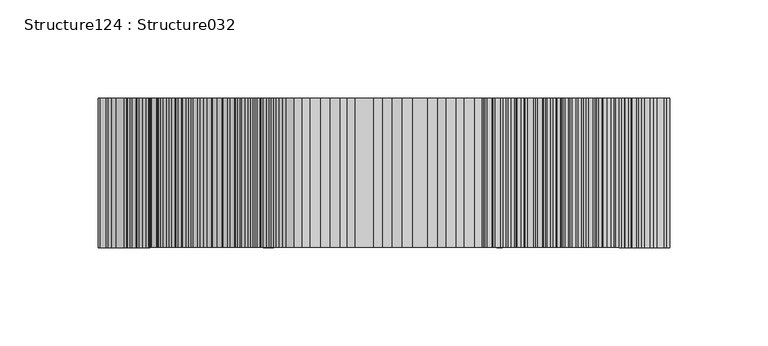
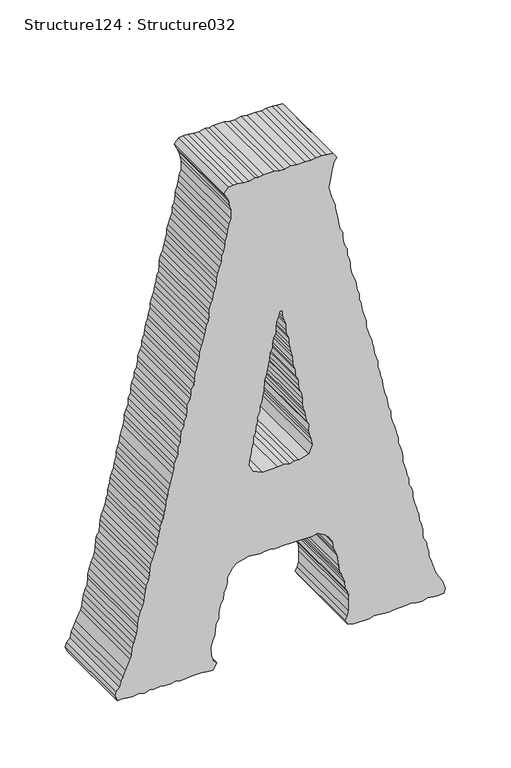
"""IFC4 building model written with IfcOpenShell, lengths in millimetres: proxy geometry, Structure124 : Structure032."""

from ifc_helpers import new_model, si_unit, frame, origin, place, context, project, spatial, polyline, outline, extrude, source, transform, mapped, element, save


def structure124_structure032_16c82b9b(model_context):
    return source(origin(), model_context, "Body", "SweptSolid", [
        extrude(outline(polyline([(3818.8310229, -39965.9490603), (3814.7296538, -39965.9490603), (3811.2043377, -39967.1091894), (3805.9476534, -39969.4487027), (3801.8462843, -39969.4487027), (3795.960595, -39970.0279649), (3791.8865042, -39972.3899428), (3787.7867397, -39972.3899428), (3783.0868532, -39974.7310607), (3777.8285642, -39975.3327874), (3773.11905, -39975.3327874), (3769.6274306, -39977.6498363), (3763.759392, -39977.6498363), (3759.6596275, -39979.4100874), (3755.559863, -39981.1719432), (3750.8583719, -39981.1719432), (3746.1745313, -39982.3529321), (3737.400554, -39984.669981), (3732.1149867, -39985.8509699), (3727.4311462, -39987.0319588), (3723.3313817, -39988.2129477), (3718.6571688, -39988.2129477), (3713.3555556, -39989.9748034), (3709.2718371, -39990.5540657), (3704.5879966, -39992.2918523), (3701.0723082, -39993.4728412), (3695.786741, -39994.0521035), (3690.512406, -39995.8139592), (3685.8285655, -39995.8139592), (3682.8857208, -39996.9949481), (3677.6274319, -39998.175937), (3672.9435914, -39999.9137237), (3668.8261762, -40001.6739748), (3664.1423357, -40002.253237), (3660.0682449, -40002.8549637), (3654.1841602, -40003.4358305), (3650.1004418, -40005.7978084), (3645.9830266, -40006.3770706), (3641.2991861, -40006.9338683), (3636.0408972, -40007.535595), (3631.915459, -40008.7165839), (3627.8397636, -40010.4768351), (3622.555801, -40012.2386908), (3617.2718384, -40013.3972153), (3613.772196, -40013.3972153), (3607.8961343, -40013.9989419), (3604.3964919, -40015.7367286), (3600.2967274, -40016.9177175), (3595.5872132, -40018.0778466), (3589.7544759, -40018.6795733), (3586.2115092, -40019.8605622), (3577.4535778, -40023.9378622), (3572.1423369, -40026.3014446), (3568.6426945, -40028.0616957), (3563.366755, -40029.1977557), (3560.441561, -40032.1389958), (3556.3417965, -40033.3215893), (3551.6675836, -40031.5597335), (3551.6675836, -40026.8807068), (3551.0658569, -40022.1776111), (3550.4833855, -40018.0778466), (3551.6675836, -40012.817953), (3550.4833855, -40007.535595), (3551.6675836, -40002.8549637), (3551.0658569, -39999.3344615), (3551.6675836, -39993.4728412), (3551.0658569, -39989.9748034), (3551.0658569, -39984.0907187), (3551.6675836, -39979.9893497), (3551.0658569, -39975.9120496), (3551.0658569, -39971.2089539), (3551.6675836, -39966.5299271), (3551.6675836, -39957.1462001), (3551.0658569, -39952.4671733), (3550.4833855, -39947.1848153), (3556.3417965, -39943.6851729), (3559.2669905, -39946.6055531), (3565.1254015, -39948.3658043), (3572.7440636, -39948.9450665), (3578.6104977, -39947.1848153), (3582.7102621, -39945.4470287), (3587.3860796, -39944.845302), (3592.0955938, -39944.2660398), (3596.7698067, -39941.9024573), (3601.4536473, -39941.9024573), (3604.9709403, -39941.3231951), (3610.2292293, -39940.1422062), (3613.772196, -39937.8251573), (3619.6145609, -39937.2458951), (3622.555801, -39935.4615749), (3627.8397636, -39934.3030505), (3633.0980525, -39934.3030505), (3639.5405396, -39929.6240237), (3643.0578326, -39926.1019169), (3644.8245022, -39919.0593077), (3645.9830266, -39915.5612699), (3645.4262289, -39909.6771853), (3644.8245022, -39905.5982806), (3645.4262289, -39900.9192539), (3645.9830266, -39896.2161581), (3644.8245022, -39892.1163937), (3645.4262289, -39886.8340357), (3645.4262289, -39874.531533), (3644.8245022, -39868.6699128), (3644.8245022, -39859.2877903), (3645.9830266, -39854.6087636), (3642.4833842, -39848.1678811), (3638.9580681, -39844.066512), (3633.0980525, -39841.1477365), (3627.2396415, -39839.9667475), (3622.555801, -39838.2048918), (3619.6145609, -39837.0239029), (3609.0723094, -39835.8653785), (3604.3964919, -39834.6843895), (3600.2967274, -39833.5258651), (3596.1953583, -39831.7640094), (3592.0955938, -39830.5830205), (3586.2115092, -39830.0037582), (3582.7102621, -39828.2435071), (3578.6104977, -39827.0625182), (3573.9266571, -39827.0625182), (3563.9412034, -39827.0625182), (3559.2669905, -39828.2435071), (3555.7416744, -39830.0037582), (3551.6675836, -39827.6642449), (3550.4833855, -39822.3818869), (3550.4833855, -39808.9208598), (3551.6675836, -39804.7986308), (3551.0658569, -39799.5387373), (3550.4833855, -39794.858106), (3550.4833855, -39790.735877), (3551.0658569, -39784.8967213), (3551.0658569, -39780.7969568), (3551.6675836, -39776.093861), (3551.6675836, -39771.9924919), (3550.4833855, -39767.3134652), (3550.4833855, -39762.0311072), (3551.6675836, -39757.3504759), (3551.0658569, -39752.0697225), (3550.4833855, -39748.5700801), (3551.0658569, -39742.7084599), (3555.1848766, -39741.5274709), (3560.441561, -39743.2893267), (3563.366755, -39744.4478511), (3568.6426945, -39747.9683534), (3572.1423369, -39749.7286045), (3576.2693797, -39751.5129247), (3586.2115092, -39754.4092358), (3590.3289243, -39756.169487), (3594.4286888, -39756.169487), (3599.1125293, -39757.3504759), (3604.3964919, -39758.5330694), (3608.4705827, -39760.8501183), (3612.5976255, -39761.451845), (3617.2718384, -39761.451845), (3622.555801, -39762.6328339), (3627.2396415, -39764.393085), (3632.5155811, -39764.9723472), (3636.0408972, -39766.1549407), (3640.114988, -39767.3134652), (3645.4262289, -39769.0737163), (3650.6845178, -39770.2322408), (3655.3587307, -39770.2322408), (3659.4584952, -39771.4132297), (3663.5598643, -39773.7768121), (3668.8261762, -39773.7768121), (3673.5276674, -39775.5145988), (3677.0449605, -39776.093861), (3682.8857208, -39777.8541121), (3686.4030139, -39779.035101), (3691.0868544, -39779.035101), (3695.2122926, -39779.6143633), (3699.8881101, -39780.7969568), (3705.7545441, -39783.1140057), (3710.4560353, -39783.1140057), (3714.5301261, -39784.2949946), (3718.0554422, -39785.4759835), (3723.3313817, -39786.6569724), (3727.4311462, -39788.4188281), (3732.7167134, -39789.5773526), (3737.9750024, -39789.5773526), (3740.9162424, -39791.3376037), (3745.6000829, -39792.4961281), (3751.4424479, -39793.0978548), (3756.1423345, -39794.858106), (3759.6596275, -39796.0406995), (3764.3611187, -39796.6199617), (3769.0176809, -39797.1767595), (3774.3032481, -39798.9370106), (3777.8285642, -39799.5387373), (3783.0868532, -39801.2989884), (3788.3611881, -39801.2989884), (3791.8865042, -39802.4799773), (3797.1463977, -39804.2193686), (3801.8462843, -39804.7986308), (3806.5317294, -39805.9796197), (3810.0474179, -39806.5588819), (3815.3313805, -39808.9208598), (3820.015221, -39810.0809888), (3824.1149855, -39811.2619777), (3829.374879, -39811.2619777), (3837.6000817, -39814.1807533), (3842.8583706, -39815.3617422), (3846.9757858, -39815.9410044), (3851.6612309, -39817.7028602), (3856.9179152, -39817.7028602), (3861.0192843, -39819.4406468), (3866.3032469, -39820.0423735), (3869.8189354, -39820.6216357), (3873.9203044, -39822.3818869), (3878.5784713, -39824.142138), (3883.8881076, -39825.3247315), (3888.5623205, -39825.3247315), (3892.6636896, -39826.5057204), (3897.3475301, -39828.2435071), (3902.6314927, -39828.2435071), (3906.1487857, -39830.5830205), (3910.8310217, -39831.7640094), (3916.0909152, -39832.3448762), (3919.6066036, -39832.3448762), (3924.2888396, -39834.6843895), (3928.9919353, -39835.8653785), (3934.2758979, -39836.4446407), (3938.9517154, -39837.6256296), (3944.235678, -39838.8066185), (3947.1496398, -39838.8066185), (3956.5349715, -39842.3062609), (3961.794865, -39843.4647853), (3965.8930249, -39844.6457743), (3974.7055128, -39842.8855231), (3979.9621971, -39841.7045342), (3983.4794902, -39841.1477365), (3987.5792547, -39839.9667475), (3991.6806238, -39837.6256296), (3996.390138, -39841.1477365), (3996.9645864, -39846.4060254), (3997.5486624, -39850.5073945), (3997.5486624, -39855.7897525), (3996.390138, -39859.889517), (3996.9645864, -39865.1494105), (3996.9645864, -39872.7712819), (3997.5486624, -39878.0536399), (3996.390138, -39883.3343933), (3996.390138, -39888.0150246), (3997.5486624, -39892.6956559), (3997.5486624, -39902.0553139), (3996.9645864, -39906.1775429), (3997.5486624, -39909.6771853), (3996.390138, -39914.9595433), (3996.390138, -39919.63857), (3997.5486624, -39924.920928), (3997.5486624, -39929.0222971), (3996.9645864, -39933.1220615), (3992.2614906, -39937.2458951), (3987.5792547, -39934.8823127), (3984.0635662, -39933.1220615), (3979.3781211, -39931.9410726), (3974.7055128, -39930.7825482), (3966.5043792, -39930.7825482), (3962.3757319, -39932.5427993), (3957.1190475, -39933.7013238), (3952.435207, -39934.3030505), (3947.7337158, -39936.0633016), (3944.235678, -39936.0633016), (3938.3499888, -39937.2458951), (3934.8503464, -39939.0061462), (3929.5904528, -39939.0061462), (3924.8905662, -39940.7439329), (3919.6066036, -39942.504184), (3915.5068392, -39943.6851729), (3910.8310217, -39943.6851729), (3906.1487857, -39944.845302), (3902.6314927, -39946.0262909), (3896.763454, -39947.1848153), (3893.822214, -39948.9450665), (3888.5623205, -39950.1260554), (3884.4609514, -39950.1260554), (3878.5784713, -39950.7053176), (3875.0772243, -39952.4671733), (3870.4030114, -39953.0464356), (3866.3032469, -39954.20496), (3861.0192843, -39955.3859489), (3856.9179152, -39956.5669378), (3851.6612309, -39958.327189), (3846.9757858, -39958.327189), (3841.6741725, -39960.0890447), (3838.1761347, -39960.6683069), (3833.4730389, -39962.4060936), (3828.2163546, -39963.0078203), (3824.1149855, -39963.5870825), (3818.8310229, -39965.9490603)]), holes=[polyline([(3720.4158154, -39903.2363028), (3723.9154578, -39911.4374364), (3730.9323932, -39914.9595433), (3736.7988273, -39913.7994142), (3741.5003184, -39912.6184253), (3744.9999608, -39912.6184253), (3750.3015741, -39910.8581742), (3755.559863, -39910.8581742), (3759.0595054, -39909.097923), (3764.3611187, -39908.5186608), (3768.4432325, -39907.3601364), (3773.11905, -39907.3601364), (3777.8285642, -39904.9965539), (3783.0868532, -39904.9965539), (3786.0280932, -39903.2363028), (3790.7039107, -39902.6570406), (3795.4037973, -39901.4985161), (3804.7730829, -39900.9192539), (3810.0474179, -39899.1573982), (3814.7296538, -39898.5556715), (3818.8310229, -39897.3746826), (3822.932392, -39896.7954204), (3828.790803, -39896.2161581), (3833.4730389, -39893.8766448), (3836.9919366, -39893.8766448), (3842.2758992, -39893.2973826), (3845.8012153, -39890.9338001), (3851.0595042, -39890.9338001), (3855.7353217, -39890.3545379), (3860.4432313, -39888.5942868), (3865.1190488, -39887.4132979), (3864.5446004, -39885.6755112), (3860.4432313, -39885.6755112), (3856.3161885, -39884.4945223), (3851.6612309, -39882.7326666), (3846.3772683, -39882.7326666), (3842.2758992, -39882.1534043), (3837.6000817, -39879.7914265), (3832.8921721, -39879.7914265), (3828.790803, -39879.2121643), (3824.1149855, -39878.0536399), (3819.4150989, -39876.8935108), (3813.5743386, -39876.2917841), (3810.0474179, -39875.7125219), (3805.9476534, -39873.9522708), (3800.6717138, -39873.9522708), (3795.4037973, -39871.6127574), (3790.7039107, -39871.6127574), (3786.0280932, -39870.4317685), (3782.5027771, -39868.6699128), (3777.2444882, -39868.0906505), (3772.5606477, -39868.0906505), (3767.8607611, -39867.5113883), (3763.759392, -39865.7511372), (3759.6596275, -39865.1494105), (3754.9854146, -39864.5701483), (3750.8583719, -39862.2306349), (3744.9999608, -39862.8323616), (3740.9162424, -39861.6497681), (3736.7988273, -39860.4687792), (3730.9323932, -39859.2877903), (3723.3313817, -39862.2306349), (3720.4158154, -39871.0334952), (3720.9726131, -39875.1107952), (3719.8140887, -39879.2121643), (3720.9726131, -39884.4945223), (3720.4158154, -39889.7752757), (3720.4158154, -39903.2363028)])]), frame((0.0, 247945.1599557, 0.0), z_axis=(0.0, 1.0, 0.0), x_axis=(0.0, 0.0, 1.0)), (0.0, 0.0, 1.0), 76.2),
    ])


if __name__ == "__main__":
    model = new_model("IFC4")
    model_context = context("Model", 3, world=origin())
    ifc_project = project(units=[si_unit("LENGTHUNIT", "METRE", prefix="MILLI")], contexts=[model_context])
    site = spatial("IfcSite", under=ifc_project)
    building = spatial("IfcBuilding", under=site)
    placement = place(None, origin())
    structure124_structure032_shape = structure124_structure032_16c82b9b(model_context)
    element("IfcBuildingElementProxy", 1, Name="Structure124 : Structure032", ObjectType="Structure124 : Structure032", at=placement, inside=building, context=model_context, shape_type="MappedRepresentation", body=[
        mapped(structure124_structure032_shape, transform((0.0, 0.0, 0.0), x_axis=(1.0, 0.0, 0.0), y_axis=(0.0, 1.0, 0.0), z_axis=(0.0, 0.0, 1.0))),
    ])
    save(model, "model.ifc")

# Revit data of these elements
# Type "Structure124 : Structure032"
#   NameOverride = "Structure032"
# Element 1 (IfcBuildingElementProxy, "Structure124 : Structure032")
#   Materials on its faces: "BRUSHED ALUM. LETTERING"
# Materials
#   "BRUSHED ALUM. LETTERING": class "Unassigned", colour RGB 169 181 186, transparency 0, Cost = 0
